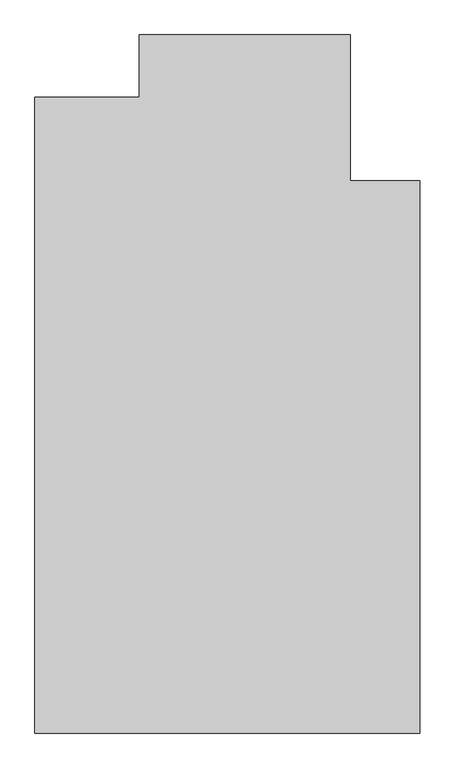
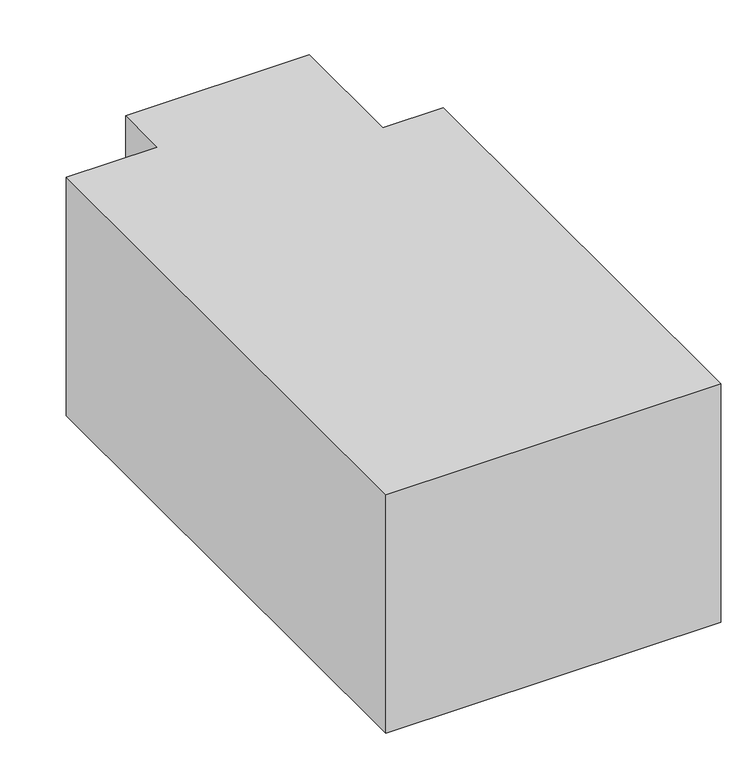
"""IFC4 building model written with IfcOpenShell, lengths in millimetres: proxy geometry, 0_3d."""

from ifc_helpers import new_model, si_unit, origin, origin_with_axes, place, context, project, spatial, polyline, outline, extrude, source, transform, mapped, element, save


def generic_models_cd385601(model_context):
    return source(origin(), model_context, "Body", "SweptSolid", [
        extrude(outline(polyline([(0.0, 0.0), (0.0, 5485.0), (900.0, 5485.0), (900.0, 6025.0), (2720.0, 6025.0), (2720.0, 4765.0), (3320.0, 4765.0), (3320.0, 0.0), (0.0, 0.0)])), origin_with_axes(), (0.0, 0.0, 1.0), 2500.0),
    ])


if __name__ == "__main__":
    model = new_model("IFC4")
    model_context = context("Model", 3, world=origin())
    ifc_project = project(units=[si_unit("LENGTHUNIT", "METRE", prefix="MILLI")], contexts=[model_context])
    site = spatial("IfcSite", under=ifc_project)
    building = spatial("IfcBuilding", under=site)
    placement = place(None, origin())
    generic_models_shape = generic_models_cd385601(model_context)
    element("IfcBuildingElementProxy", 1, Name="0_3d", ObjectType="0_3d", at=placement, inside=building, context=model_context, shape_type="MappedRepresentation", body=[
        mapped(generic_models_shape, transform((0.0, 0.0, 0.0), x_axis=(1.0, 0.0, 0.0), y_axis=(0.0, 1.0, 0.0), z_axis=(0.0, 0.0, 1.0))),
    ])
    save(model, "model.ifc")

# Revit data of these elements
# Element 1 (IfcBuildingElementProxy, "0_3d")
#   Materials on its faces: "*1"
# Materials
#   "*1": class "Unassigned", colour RGB 175 175 175, transparency 0
